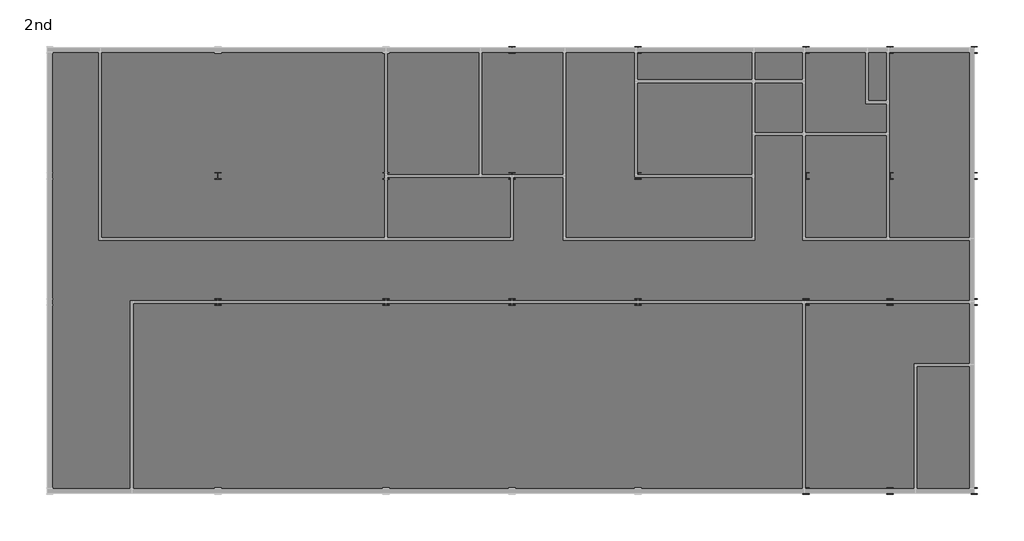
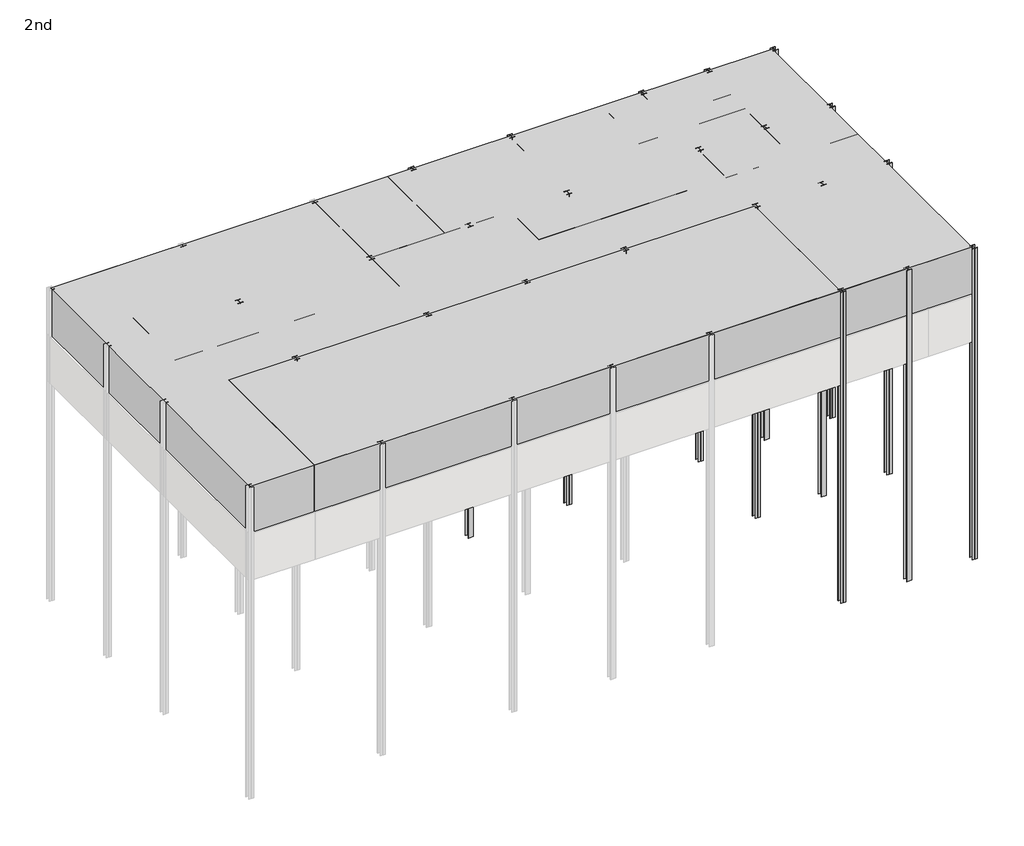
# One storey, part 3 of 3: 17 proxies, 16 columns.
# Revit data of these elements (continued)
# Element 15 (IfcBuildingElementProxy, "Space Planning Box_hec : Space Planning Box_hec") (continued)
#   Room Name = "Engineer Room"
#   Interior Finish = "IF3"
#   Exterior Finish = "EF1"
#   Department = "CI"
#   Width = 9000 mm
#   Program Area = 120 m²
#   Length = 13600 mm
#   Height = 6000 mm
#   Area = 122.4 m²
#   Fill Color = Lime
#   Phase Created = New Construction
#   Materials on its faces: "Lime"
# Element 16 (IfcBuildingElementProxy, "Space Planning Box_hec : Space Planning Box_hec")
#   Room Name = "Fire Gas Room"
#   Interior Finish = "IF1"
#   Exterior Finish = "EF1"
#   Department = "SF"
#   Width = 8000 mm
#   Program Area = 0 m²
#   Length = 9000 mm
#   Height = 6000 mm
#   Area = 72 m²
#   Fill Color = Cyan
#   Phase Created = New Construction
#   Materials on its faces: "Cyan"
# Element 17 (IfcBuildingElementProxy, "Space Planning Box_hec : Space Planning Box_hec")
#   Room Name = "Corridor"
#   Interior Finish = "IF2-1"
#   Exterior Finish = "EF1"
#   Department = "AR"
#   Width = 43900 mm
#   Program Area = 0 m²
#   Length = 21000 mm
#   Height = 6000 mm
#   Area = 921.9 m²
#   Fill Color = Lavender
#   Phase Created = New Construction
#   Materials on its faces: "Lavender"
# Elements 18, 19, 20, 21, 22, 23, 24, 25, 26, 27, 28, 29, 30, 31, 32, 33 (IfcColumn, "UC-Universal Columns-Column : UC305x305x97")
#   Structural Material = Metal - Steel 43-275
#   Phase Created = New Construction
#   Materials on its faces: "Metal - Steel 43-275"
# Materials
#   "Cyan": class "Generic", colour RGB 0 255 255, transparency 0.2, Cost = 0
#   "Metal - Steel 43-275": class "Metal", colour RGB 247 247 247, transparency 0, Cost = 0
#   "Lavender": class "Generic", colour RGB 186 85 211, transparency 0.2, Cost = 0
#   "Pink": class "Generic", colour RGB 255 105 180, transparency 0.2, Cost = 0
#   "Lime": class "Generic", colour RGB 0 255 0, transparency 0.2, Cost = 0
